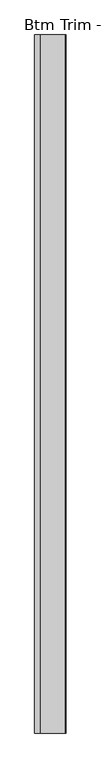
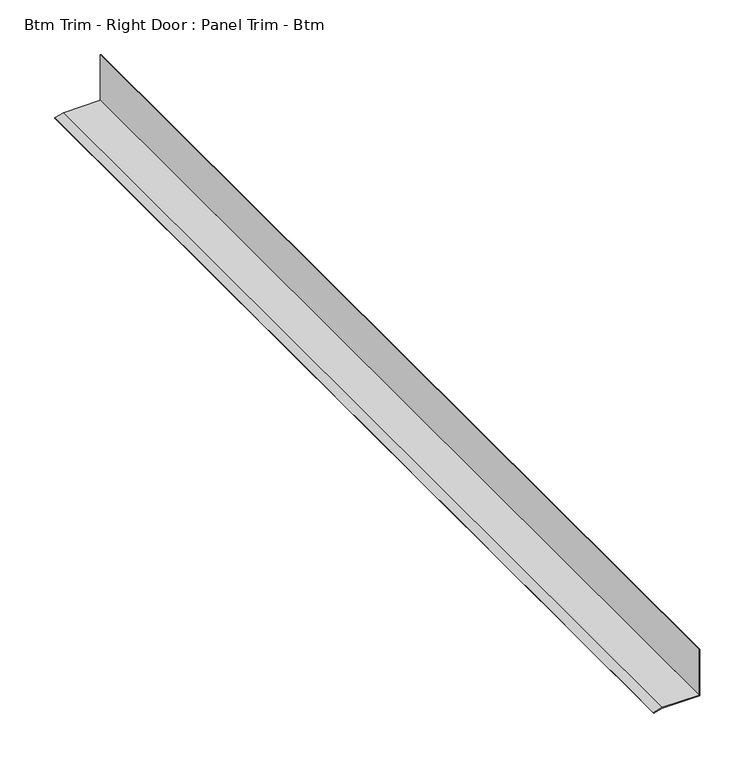
"""IFC4 building model written with IfcOpenShell, lengths in millimetres: proxy geometry, Btm Trim - Right Door : Panel Trim - Btm."""

import ifcopenshell
import ifcopenshell.guid

model = None  # the IFC model being written
_history = None  # IfcOwnerHistory: only IFC2X3 demands one
_inside = {}  # id of a spatial element -> (the spatial element, [elements in it])
_under = {}  # id of a project, library or spatial element -> (it, [spatial elements below it])
_declared = {}  # id of a project -> (the project, [libraries it declares])
_typed = {}  # id of a type object -> (the type object, [elements of that type])
_made_of = {}  # id of a material, layer set ... -> (it, [elements and type objects made of it])


def new_model(schema):
    """Start an empty IFC model of exactly this schema.

    Asked for "IFC4X3", IfcOpenShell would pick the latest addendum, in which some entities
    have other attributes; the version numbers below select the first issue.
    IFC2X3 requires an IfcOwnerHistory on every rooted entity: one is made here for all.
    """
    global model, _history
    if schema == "IFC4X3":
        model = ifcopenshell.file(schema_version=(4, 3, 0, 0))
    else:
        model = ifcopenshell.file(schema=schema)
    _inside.clear()
    _under.clear()
    _declared.clear()
    _typed.clear()
    _made_of.clear()
    _history = None
    if model.schema == "IFC2X3":
        org = make("IfcOrganization", Name="unknown")
        user = make(
            "IfcPersonAndOrganization",
            ThePerson=make("IfcPerson", FamilyName="unknown"),
            TheOrganization=org,
        )
        app = make(
            "IfcApplication",
            ApplicationDeveloper=org,
            Version="unknown",
            ApplicationFullName="unknown",
            ApplicationIdentifier="unknown",
        )
        _history = make(
            "IfcOwnerHistory",
            OwningUser=user,
            OwningApplication=app,
            ChangeAction="ADDED",
            CreationDate=0,
        )
    return model


def make(cls, **values):
    """One entity of the class cls with the attributes given. An attribute that is None is left unset."""
    return model.create_entity(
        cls, **{name: value for name, value in values.items() if value is not None}
    )


def rooted(cls, **values):
    """An entity with a GlobalId (a new one), such as an element, a storey or a relation."""
    return make(cls, GlobalId=ifcopenshell.guid.new(), OwnerHistory=_history, **values)


def si_unit(unit_type, name, prefix=None):
    """IfcSIUnit, for example si_unit("LENGTHUNIT", "METRE", prefix="MILLI")."""
    return make("IfcSIUnit", UnitType=unit_type, Prefix=prefix, Name=name)


def assignment(units):
    """IfcUnitAssignment: the units of a project."""
    return None if units is None else make("IfcUnitAssignment", Units=units)


def point(xyz):
    """IfcCartesianPoint."""
    return None if xyz is None else make("IfcCartesianPoint", Coordinates=xyz)


def direction(xyz):
    """IfcDirection."""
    return None if xyz is None else make("IfcDirection", DirectionRatios=xyz)


def frame(location, z_axis=None, x_axis=None):
    """IfcAxis2Placement3D, a coordinate frame: its origin and axes. An axis left out is left unset."""
    return make(
        "IfcAxis2Placement3D",
        Location=point(location),
        Axis=direction(z_axis),
        RefDirection=direction(x_axis),
    )


def origin():
    """The frame at (0, 0, 0) with its axes left unset."""
    return frame((0.0, 0.0, 0.0))


def place(relative_to, where):
    """IfcLocalPlacement: puts the frame where relative to a parent placement (None: the world)."""
    return make(
        "IfcLocalPlacement", PlacementRelTo=relative_to, RelativePlacement=where
    )


def context(
    kind, dimensions, precision=None, world=None, true_north=None, identifier=None
):
    """IfcGeometricRepresentationContext, for example the 3D "Model" context."""
    return make(
        "IfcGeometricRepresentationContext",
        ContextIdentifier=identifier,
        ContextType=kind,
        CoordinateSpaceDimension=dimensions,
        Precision=precision,
        WorldCoordinateSystem=world,
        TrueNorth=true_north,
    )


def project(units=None, contexts=None):
    """IfcProject with its units and contexts."""
    return rooted(
        "IfcProject",
        Name="project",
        RepresentationContexts=contexts,
        UnitsInContext=assignment(units),
    )


def spatial(cls, under=None, at=None, **own):
    """A site, building, storey or space (cls), placed at a placement, below another one or the project."""
    s = rooted(cls, ObjectPlacement=at, **own)
    if under is not None:
        _under.setdefault(under.id(), (under, []))[1].append(s)
    return s


def polyline(points):
    """IfcPolyline through the points."""
    return make("IfcPolyline", Points=[point(p) for p in points])


def outline(outer, holes=None, kind="AREA"):
    """IfcArbitraryClosedProfileDef: a profile drawn as a closed curve; with holes, ...WithVoids."""
    if holes is None:
        return make("IfcArbitraryClosedProfileDef", ProfileType=kind, OuterCurve=outer)
    return make(
        "IfcArbitraryProfileDefWithVoids",
        ProfileType=kind,
        OuterCurve=outer,
        InnerCurves=holes,
    )


def extrude(swept, where, along, depth):
    """IfcExtrudedAreaSolid: the profile swept, set in the frame where, extruded along a direction by depth."""
    return make(
        "IfcExtrudedAreaSolid",
        SweptArea=swept,
        Position=where,
        ExtrudedDirection=direction(along),
        Depth=depth,
    )


def shape(context_of_items, identifier, shape_type, items):
    """IfcShapeRepresentation: the items that make up one representation, for example the "Body"."""
    return make(
        "IfcShapeRepresentation",
        ContextOfItems=context_of_items,
        RepresentationIdentifier=identifier,
        RepresentationType=shape_type,
        Items=items,
    )


def source(mapping_origin, context_of_items, identifier, shape_type, items):
    """IfcRepresentationMap: a shape defined once, which mapped items show again and again."""
    return make(
        "IfcRepresentationMap",
        MappingOrigin=mapping_origin,
        MappedRepresentation=shape(context_of_items, identifier, shape_type, items),
    )


def transform(
    local_origin,
    x_axis=None,
    y_axis=None,
    z_axis=None,
    scale=None,
    scale2=None,
    scale3=None,
    uniform=True,
):
    """IfcCartesianTransformationOperator3D, or its non-uniform kind. x_axis, y_axis, z_axis: its Axis1, 2, 3."""
    if uniform:
        return make(
            "IfcCartesianTransformationOperator3D",
            Axis1=direction(x_axis),
            Axis2=direction(y_axis),
            LocalOrigin=point(local_origin),
            Scale=scale,
            Axis3=direction(z_axis),
        )
    return make(
        "IfcCartesianTransformationOperator3DnonUniform",
        Axis1=direction(x_axis),
        Axis2=direction(y_axis),
        LocalOrigin=point(local_origin),
        Scale=scale,
        Axis3=direction(z_axis),
        Scale2=scale2,
        Scale3=scale3,
    )


def mapped(mapping_source, mapping_target):
    """IfcMappedItem: shows the shape of a source again, moved by a transform."""
    return make(
        "IfcMappedItem", MappingSource=mapping_source, MappingTarget=mapping_target
    )


def made_of(thing, what):
    """Note that an element or type object is made of a material, layer set ...; save() writes the relation."""
    if what is not None:
        _made_of.setdefault(what.id(), (what, []))[1].append(thing)
    return thing


def element(
    cls,
    number,
    at=None,
    inside=None,
    cuts=None,
    type_object=None,
    material=None,
    context=None,
    identifier="Body",
    shape_type=None,
    held_by="IfcProductDefinitionShape",
    body=None,
    shapes=None,
    **own,
):
    """One element of the class cls, such as IfcWall. Its Tag is "e" and its number.

    at: its placement. inside: the storey or other place that contains it. cuts: it is an
    opening in that element (IfcRelVoidsElement). A single representation is given by context,
    identifier, shape_type and body (its items); several are given by shapes. held_by: the class
    of the entity that holds the representations. save() writes the other relations.
    """
    e = rooted(cls, Tag="e%d" % number, ObjectPlacement=at, **own)
    if body is not None:
        shapes = [shape(context, identifier, shape_type, body)]
    if shapes is not None:
        e.Representation = make(held_by, Representations=shapes)
    if inside is not None:
        _inside.setdefault(inside.id(), (inside, []))[1].append(e)
    if cuts is not None:
        rooted(
            "IfcRelVoidsElement", RelatingBuildingElement=cuts, RelatedOpeningElement=e
        )
    if type_object is not None:
        _typed.setdefault(type_object.id(), (type_object, []))[1].append(e)
    return made_of(e, material)


def aggregate(whole, parts):
    """IfcRelAggregates: a whole, such as a stair, and the parts it consists of."""
    return rooted("IfcRelAggregates", RelatingObject=whole, RelatedObjects=parts)


def save(model, path):
    """Write the relations noted so far, then the file.

    IfcRelAggregates (storeys below a building ...), IfcRelContainedInSpatialStructure (elements
    in a storey), IfcRelDefinesByType, IfcRelAssociatesMaterial and IfcRelDeclares: one each for
    every whole, place, type object, material and project.
    """
    for whole, parts in _under.values():
        aggregate(whole, parts)
    for where, things in _inside.values():
        rooted(
            "IfcRelContainedInSpatialStructure",
            RelatedElements=things,
            RelatingStructure=where,
        )
    for kind, things in _typed.values():
        rooted("IfcRelDefinesByType", RelatedObjects=things, RelatingType=kind)
    for what, things in _made_of.values():
        rooted("IfcRelAssociatesMaterial", RelatedObjects=things, RelatingMaterial=what)
    for by, libraries in _declared.values():
        rooted("IfcRelDeclares", RelatingContext=by, RelatedDefinitions=libraries)
    model.write(path)


def btm_trim_right_door_panel_trim_btm_5f1d7bb7(model_context):
    return source(origin(), model_context, "Body", "SweptSolid", [
        extrude(outline(polyline([(50.8, 587326.1141748), (48.3077022, 587316.8127928), (47.5409986, 587317.0182304), (50.00625, 587326.2186739), (50.00625, 587365.8934739), (101.6, 587365.8934739), (101.6, 587365.1060739), (50.8, 587365.1060739), (50.8, 587326.1141748)])), frame((0.0, -533977.6038841, 0.0), z_axis=(0.0, 1.0, 0.0), x_axis=(0.0, 0.0, 1.0)), (0.0, 0.0, 1.0), 1094.5749),
    ])


if __name__ == "__main__":
    model = new_model("IFC4")
    model_context = context("Model", 3, world=origin())
    ifc_project = project(units=[si_unit("LENGTHUNIT", "METRE", prefix="MILLI")], contexts=[model_context])
    site = spatial("IfcSite", under=ifc_project)
    building = spatial("IfcBuilding", under=site)
    placement = place(None, origin())
    btm_trim_right_door_panel_trim_btm_shape = btm_trim_right_door_panel_trim_btm_5f1d7bb7(model_context)
    element("IfcBuildingElementProxy", 1, Name="Btm Trim - Right Door : Panel Trim - Btm", ObjectType="Btm Trim - Right Door : Panel Trim - Btm", at=placement, inside=building, context=model_context, shape_type="MappedRepresentation", body=[
        mapped(btm_trim_right_door_panel_trim_btm_shape, transform((0.0, 0.0, 0.0), x_axis=(1.0, 0.0, 0.0), y_axis=(0.0, 1.0, 0.0), z_axis=(0.0, 0.0, 1.0))),
    ])
    save(model, "model.ifc")

# Revit data of these elements
# Element 1 (IfcBuildingElementProxy, "Btm Trim - Right Door : Panel Trim - Btm")
#   Materials on its faces: "BASE TRIM BY MTL PANEL MFR."
# Materials
#   "BASE TRIM BY MTL PANEL MFR.": class "Generic", colour RGB 239 242 240, transparency 0, Cost = 0
